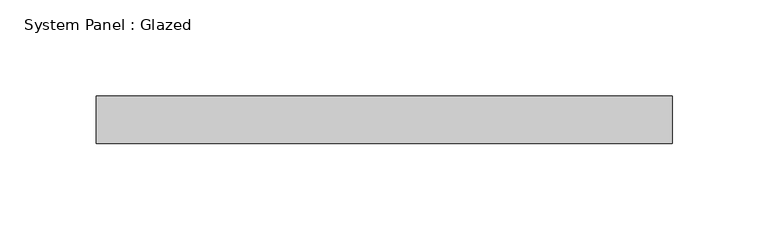
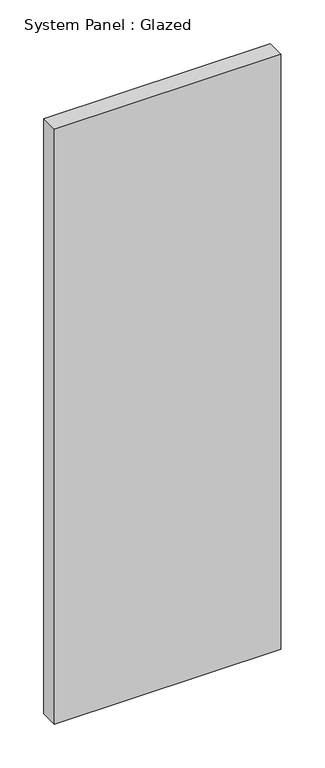
"""IFC4 building model written with IfcOpenShell, lengths in millimetres: plate geometry, System Panel : Glazed."""

from ifc_helpers import new_model, si_unit, origin, origin_with_axes, place, context, project, spatial, polyline, outline, extrude, source, transform, mapped, element, save


def system_panel_glazed_0b22f4b4(model_context):
    return source(origin(), model_context, "Body", "SweptSolid", [
        extrude(outline(polyline([(150.0, 24.5), (-150.0, 24.5), (-150.0, 49.5), (150.0, 49.5), (150.0, 24.5)])), origin_with_axes(), (0.0, 0.0, 1.0), 833.3333333),
    ])


if __name__ == "__main__":
    model = new_model("IFC4")
    model_context = context("Model", 3, world=origin())
    ifc_project = project(units=[si_unit("LENGTHUNIT", "METRE", prefix="MILLI")], contexts=[model_context])
    site = spatial("IfcSite", under=ifc_project)
    building = spatial("IfcBuilding", under=site)
    placement = place(None, origin())
    system_panel_glazed_shape = system_panel_glazed_0b22f4b4(model_context)
    element("IfcPlate", 1, ObjectType="System Panel : Glazed", at=placement, inside=building, context=model_context, shape_type="MappedRepresentation", body=[
        mapped(system_panel_glazed_shape, transform((0.0, 0.0, 0.0), x_axis=(1.0, 0.0, 0.0), y_axis=(0.0, 1.0, 0.0), z_axis=(0.0, 0.0, 1.0))),
    ])
    save(model, "model.ifc")

# Revit data of these elements
# Element 1 (IfcPlate, "System Panel : Glazed")
#   Materials on its faces: "Glass"
# Materials
#   "Glass": class "Glass", colour RGB 218 227 224, transparency 0.85, Description = "Soda Lime Glass", Cost = 0
